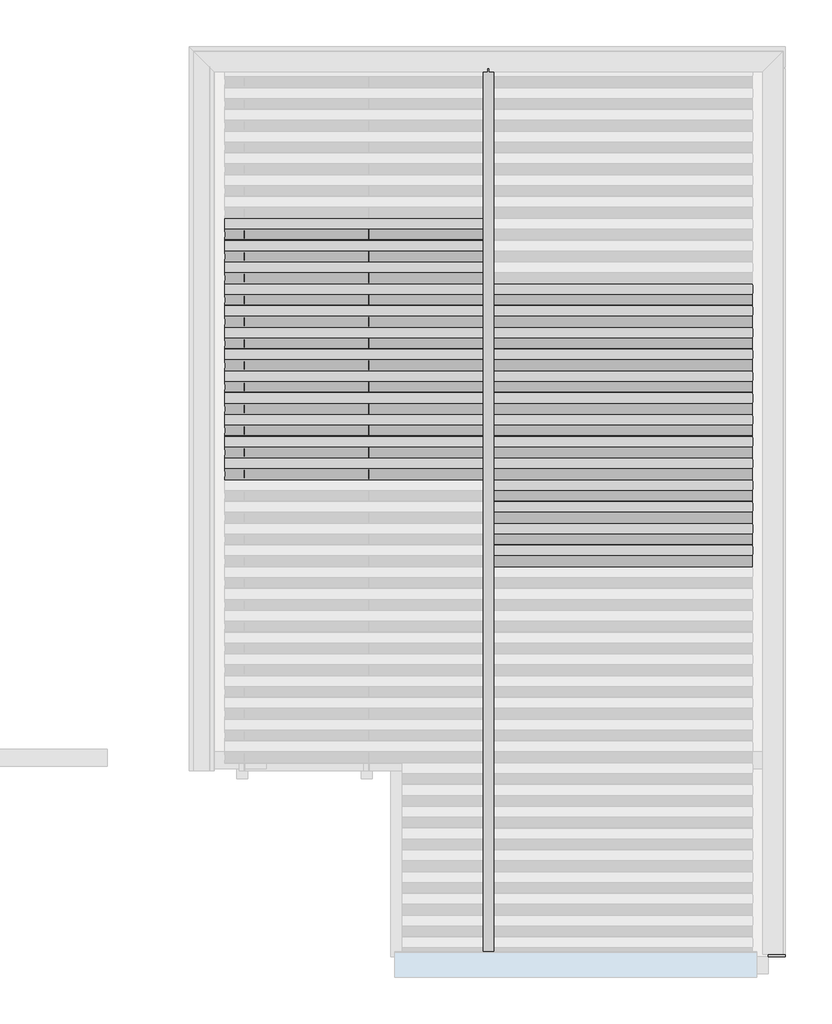
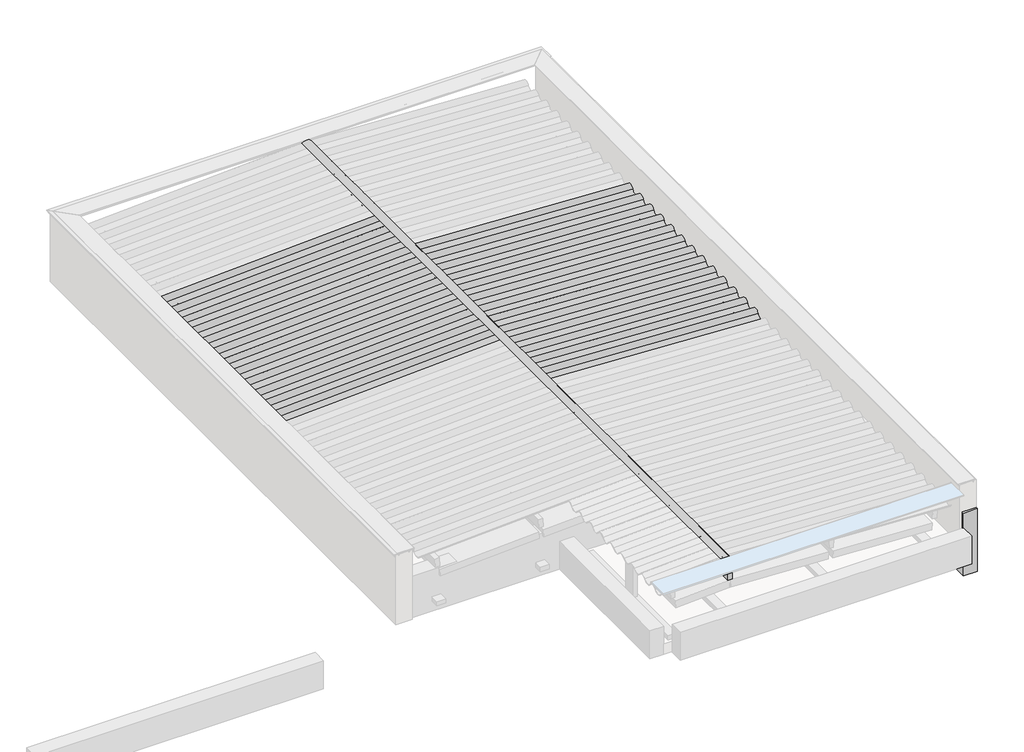
# One storey, part 3 of 4: 37 beams, 8 columns.
"""IFC4 building model written with IfcOpenShell, lengths in millimetres."""

import ifcopenshell
import ifcopenshell.guid

model = None  # the IFC model being written
_history = None  # IfcOwnerHistory: only IFC2X3 demands one
_inside = {}  # id of a spatial element -> (the spatial element, [elements in it])
_under = {}  # id of a project, library or spatial element -> (it, [spatial elements below it])
_declared = {}  # id of a project -> (the project, [libraries it declares])
_typed = {}  # id of a type object -> (the type object, [elements of that type])
_made_of = {}  # id of a material, layer set ... -> (it, [elements and type objects made of it])


def new_model(schema):
    """Start an empty IFC model of exactly this schema.

    Asked for "IFC4X3", IfcOpenShell would pick the latest addendum, in which some entities
    have other attributes; the version numbers below select the first issue.
    IFC2X3 requires an IfcOwnerHistory on every rooted entity: one is made here for all.
    """
    global model, _history
    if schema == "IFC4X3":
        model = ifcopenshell.file(schema_version=(4, 3, 0, 0))
    else:
        model = ifcopenshell.file(schema=schema)
    _inside.clear()
    _under.clear()
    _declared.clear()
    _typed.clear()
    _made_of.clear()
    _history = None
    if model.schema == "IFC2X3":
        org = make("IfcOrganization", Name="unknown")
        user = make(
            "IfcPersonAndOrganization",
            ThePerson=make("IfcPerson", FamilyName="unknown"),
            TheOrganization=org,
        )
        app = make(
            "IfcApplication",
            ApplicationDeveloper=org,
            Version="unknown",
            ApplicationFullName="unknown",
            ApplicationIdentifier="unknown",
        )
        _history = make(
            "IfcOwnerHistory",
            OwningUser=user,
            OwningApplication=app,
            ChangeAction="ADDED",
            CreationDate=0,
        )
    return model


def make(cls, **values):
    """One entity of the class cls with the attributes given. An attribute that is None is left unset."""
    return model.create_entity(
        cls, **{name: value for name, value in values.items() if value is not None}
    )


def rooted(cls, **values):
    """An entity with a GlobalId (a new one), such as an element, a storey or a relation."""
    return make(cls, GlobalId=ifcopenshell.guid.new(), OwnerHistory=_history, **values)


def si_unit(unit_type, name, prefix=None):
    """IfcSIUnit, for example si_unit("LENGTHUNIT", "METRE", prefix="MILLI")."""
    return make("IfcSIUnit", UnitType=unit_type, Prefix=prefix, Name=name)


def assignment(units):
    """IfcUnitAssignment: the units of a project."""
    return None if units is None else make("IfcUnitAssignment", Units=units)


def point(xyz):
    """IfcCartesianPoint."""
    return None if xyz is None else make("IfcCartesianPoint", Coordinates=xyz)


def direction(xyz):
    """IfcDirection."""
    return None if xyz is None else make("IfcDirection", DirectionRatios=xyz)


def frame(location, z_axis=None, x_axis=None):
    """IfcAxis2Placement3D, a coordinate frame: its origin and axes. An axis left out is left unset."""
    return make(
        "IfcAxis2Placement3D",
        Location=point(location),
        Axis=direction(z_axis),
        RefDirection=direction(x_axis),
    )


def frame_2d(location, x_axis=None):
    """IfcAxis2Placement2D, a coordinate frame in the plane: its origin and x axis."""
    return make(
        "IfcAxis2Placement2D", Location=point(location), RefDirection=direction(x_axis)
    )


def origin():
    """The frame at (0, 0, 0) with its axes left unset."""
    return frame((0.0, 0.0, 0.0))


def place(relative_to, where):
    """IfcLocalPlacement: puts the frame where relative to a parent placement (None: the world)."""
    return make(
        "IfcLocalPlacement", PlacementRelTo=relative_to, RelativePlacement=where
    )


def context(
    kind, dimensions, precision=None, world=None, true_north=None, identifier=None
):
    """IfcGeometricRepresentationContext, for example the 3D "Model" context."""
    return make(
        "IfcGeometricRepresentationContext",
        ContextIdentifier=identifier,
        ContextType=kind,
        CoordinateSpaceDimension=dimensions,
        Precision=precision,
        WorldCoordinateSystem=world,
        TrueNorth=true_north,
    )


def project(units=None, contexts=None):
    """IfcProject with its units and contexts."""
    return rooted(
        "IfcProject",
        Name="project",
        RepresentationContexts=contexts,
        UnitsInContext=assignment(units),
    )


def spatial(cls, under=None, at=None, **own):
    """A site, building, storey or space (cls), placed at a placement, below another one or the project."""
    s = rooted(cls, ObjectPlacement=at, **own)
    if under is not None:
        _under.setdefault(under.id(), (under, []))[1].append(s)
    return s


def polyline(points):
    """IfcPolyline through the points."""
    return make("IfcPolyline", Points=[point(p) for p in points])


def circle_curve(where, radius):
    """IfcCircle in the frame where."""
    return make("IfcCircle", Position=where, Radius=radius)


def trimmed(basis, trim1, trim2, sense, master):
    """IfcTrimmedCurve: the piece of a basis curve between two trims."""
    return make(
        "IfcTrimmedCurve",
        BasisCurve=basis,
        Trim1=trim1,
        Trim2=trim2,
        SenseAgreement=sense,
        MasterRepresentation=master,
    )


def segment(curve, same_sense, transition):
    """IfcCompositeCurveSegment."""
    return make(
        "IfcCompositeCurveSegment",
        Transition=transition,
        SameSense=same_sense,
        ParentCurve=curve,
    )


def composite_curve(segments, self_intersect=None):
    """IfcCompositeCurve: segments joined end to end."""
    return make("IfcCompositeCurve", Segments=segments, SelfIntersect=self_intersect)


def outline(outer, holes=None, kind="AREA"):
    """IfcArbitraryClosedProfileDef: a profile drawn as a closed curve; with holes, ...WithVoids."""
    if holes is None:
        return make("IfcArbitraryClosedProfileDef", ProfileType=kind, OuterCurve=outer)
    return make(
        "IfcArbitraryProfileDefWithVoids",
        ProfileType=kind,
        OuterCurve=outer,
        InnerCurves=holes,
    )


def extrude(swept, where, along, depth):
    """IfcExtrudedAreaSolid: the profile swept, set in the frame where, extruded along a direction by depth."""
    return make(
        "IfcExtrudedAreaSolid",
        SweptArea=swept,
        Position=where,
        ExtrudedDirection=direction(along),
        Depth=depth,
    )


def faces_of(points, faces, orient=None, outer=None):
    """IfcFace entities. A face is a list of loops; a loop is a list of indices into points, from 0.

    orient and outer hold one flag for each loop. By default every Orientation is true, the
    first loop of a face is its IfcFaceOuterBound and the others are IfcFaceBound.
    """
    made = []
    for i, loops in enumerate(faces):
        bounds = []
        for j, loop in enumerate(loops):
            is_outer = j == 0 if outer is None else outer[i][j]
            bounds.append(
                make(
                    "IfcFaceOuterBound" if is_outer else "IfcFaceBound",
                    Bound=make("IfcPolyLoop", Polygon=[points[k] for k in loop]),
                    Orientation=True if orient is None else orient[i][j],
                )
            )
        made.append(make("IfcFace", Bounds=bounds))
    return made


def faceted_brep(points, faces, orient=None, outer=None, voids=None):
    """IfcFacetedBrep: a solid bounded by flat faces; with voids (closed shells), ...WithVoids."""
    shared = [point(p) for p in points]
    hull = make("IfcClosedShell", CfsFaces=faces_of(shared, faces, orient, outer))
    if voids is None:
        return make("IfcFacetedBrep", Outer=hull)
    return make(
        "IfcFacetedBrepWithVoids",
        Outer=hull,
        Voids=[
            make(cls, CfsFaces=faces_of(shared, fs, o, b)) for cls, fs, o, b in voids
        ],
    )


def shape(context_of_items, identifier, shape_type, items):
    """IfcShapeRepresentation: the items that make up one representation, for example the "Body"."""
    return make(
        "IfcShapeRepresentation",
        ContextOfItems=context_of_items,
        RepresentationIdentifier=identifier,
        RepresentationType=shape_type,
        Items=items,
    )


def source(mapping_origin, context_of_items, identifier, shape_type, items):
    """IfcRepresentationMap: a shape defined once, which mapped items show again and again."""
    return make(
        "IfcRepresentationMap",
        MappingOrigin=mapping_origin,
        MappedRepresentation=shape(context_of_items, identifier, shape_type, items),
    )


def transform(
    local_origin,
    x_axis=None,
    y_axis=None,
    z_axis=None,
    scale=None,
    scale2=None,
    scale3=None,
    uniform=True,
):
    """IfcCartesianTransformationOperator3D, or its non-uniform kind. x_axis, y_axis, z_axis: its Axis1, 2, 3."""
    if uniform:
        return make(
            "IfcCartesianTransformationOperator3D",
            Axis1=direction(x_axis),
            Axis2=direction(y_axis),
            LocalOrigin=point(local_origin),
            Scale=scale,
            Axis3=direction(z_axis),
        )
    return make(
        "IfcCartesianTransformationOperator3DnonUniform",
        Axis1=direction(x_axis),
        Axis2=direction(y_axis),
        LocalOrigin=point(local_origin),
        Scale=scale,
        Axis3=direction(z_axis),
        Scale2=scale2,
        Scale3=scale3,
    )


def mapped(mapping_source, mapping_target):
    """IfcMappedItem: shows the shape of a source again, moved by a transform."""
    return make(
        "IfcMappedItem", MappingSource=mapping_source, MappingTarget=mapping_target
    )


def made_of(thing, what):
    """Note that an element or type object is made of a material, layer set ...; save() writes the relation."""
    if what is not None:
        _made_of.setdefault(what.id(), (what, []))[1].append(thing)
    return thing


def element(
    cls,
    number,
    at=None,
    inside=None,
    cuts=None,
    type_object=None,
    material=None,
    context=None,
    identifier="Body",
    shape_type=None,
    held_by="IfcProductDefinitionShape",
    body=None,
    shapes=None,
    **own,
):
    """One element of the class cls, such as IfcWall. Its Tag is "e" and its number.

    at: its placement. inside: the storey or other place that contains it. cuts: it is an
    opening in that element (IfcRelVoidsElement). A single representation is given by context,
    identifier, shape_type and body (its items); several are given by shapes. held_by: the class
    of the entity that holds the representations. save() writes the other relations.
    """
    e = rooted(cls, Tag="e%d" % number, ObjectPlacement=at, **own)
    if body is not None:
        shapes = [shape(context, identifier, shape_type, body)]
    if shapes is not None:
        e.Representation = make(held_by, Representations=shapes)
    if inside is not None:
        _inside.setdefault(inside.id(), (inside, []))[1].append(e)
    if cuts is not None:
        rooted(
            "IfcRelVoidsElement", RelatingBuildingElement=cuts, RelatedOpeningElement=e
        )
    if type_object is not None:
        _typed.setdefault(type_object.id(), (type_object, []))[1].append(e)
    return made_of(e, material)


def aggregate(whole, parts):
    """IfcRelAggregates: a whole, such as a stair, and the parts it consists of."""
    return rooted("IfcRelAggregates", RelatingObject=whole, RelatedObjects=parts)


def save(model, path):
    """Write the relations noted so far, then the file.

    IfcRelAggregates (storeys below a building ...), IfcRelContainedInSpatialStructure (elements
    in a storey), IfcRelDefinesByType, IfcRelAssociatesMaterial and IfcRelDeclares: one each for
    every whole, place, type object, material and project.
    """
    for whole, parts in _under.values():
        aggregate(whole, parts)
    for where, things in _inside.values():
        rooted(
            "IfcRelContainedInSpatialStructure",
            RelatedElements=things,
            RelatingStructure=where,
        )
    for kind, things in _typed.values():
        rooted("IfcRelDefinesByType", RelatedObjects=things, RelatingType=kind)
    for what, things in _made_of.values():
        rooted("IfcRelAssociatesMaterial", RelatedObjects=things, RelatingMaterial=what)
    for by, libraries in _declared.values():
        rooted("IfcRelDeclares", RelatingContext=by, RelatedDefinitions=libraries)
    model.write(path)


def cumeeira_telha_ondulada_fibrocimento_c9eafb3e(model_context):
    return source(origin(), model_context, "Body", "SweptSolid", [
        extrude(outline(composite_curve([segment(polyline([(58.3970135, 42.4437972), (53.9055884, 40.2467307)]), True, "CONTINUOUS"), segment(trimmed(circle_curve(frame_2d((-1.6029865, 13.0936483)), 61.7939461), [point((53.9055884, 40.2467307))], [point((-57.1115615, 40.2467307))], True, "CARTESIAN"), True, "CONTINUOUS"), segment(polyline([(-57.1115615, 40.2467307), (-61.6029865, 42.4437972)]), True, "CONTINUOUS"), segment(trimmed(circle_curve(frame_2d((-1.6029865, 13.0936483)), 66.7939461), [point((-61.6029865, 42.4437972))], [point((58.3970135, 42.4437972))], False, "CARTESIAN"), True, "CONTINUOUS")], self_intersect=False)), frame((-4969.5, 0.0, 0.0), z_axis=(1.0, 0.0, 0.0), x_axis=(0.0, 1.0, 0.0)), (0.0, 0.0, 1.0), 9939.0),
    ])


def viga_cumeeira_6x16cm_5eb8e513(model_context):
    return source(origin(), model_context, "Body", "SweptSolid", [
        extrude(outline(polyline([(4969.5, 30.0), (4969.5, -30.0), (-4969.5, -30.0), (-4969.5, 30.0), (4969.5, 30.0)])), frame((0.0, 0.0, -80.0), z_axis=(0.0, 0.0, 1.0), x_axis=(1.0, 0.0, 0.0)), (0.0, 0.0, 1.0), 160.0),
    ])


def column_f3930958(model_context):
    return source(origin(), model_context, "Body", "SweptSolid", [
        extrude(outline(polyline([(30.0, 80.0), (30.0, -80.0), (-30.0, -80.0), (-30.0, 80.0), (30.0, 80.0)])), frame((0.0, 0.0, 4460.0), z_axis=(0.0, 0.0, 1.0), x_axis=(1.0, 0.0, 0.0)), (0.0, 0.0, 1.0), 522.9),
    ])


def column_4d3918cc(model_context):
    return source(origin(), model_context, "Body", "SweptSolid", [
        extrude(outline(polyline([(30.0, 80.0), (30.0, -80.0), (-30.0, -80.0), (-30.0, 80.0), (30.0, 80.0)])), frame((0.0, 0.0, 4460.0), z_axis=(0.0, 0.0, 1.0), x_axis=(1.0, 0.0, 0.0)), (0.0, 0.0, 1.0), 426.9),
    ])


def column_924cc83b(model_context):
    return source(origin(), model_context, "Body", "SweptSolid", [
        extrude(outline(polyline([(30.0, 80.0), (30.0, -80.0), (-30.0, -80.0), (-30.0, 80.0), (30.0, 80.0)])), frame((0.0, 0.0, 4460.0), z_axis=(0.0, 0.0, 1.0), x_axis=(1.0, 0.0, 0.0)), (0.0, 0.0, 1.0), 497.0),
    ])


model = new_model("IFC4")

# Units and contexts
model_context = context("Model", 3, world=origin())
ifc_project = project(units=[si_unit("LENGTHUNIT", "METRE", prefix="MILLI")], contexts=[model_context])

# Site, building, storey
site = spatial("IfcSite", under=ifc_project)
building = spatial("IfcBuilding", under=site)
storey = spatial("IfcBuildingStorey", under=building, Name="COB. SALA ESTAR", Elevation=4400.0)

# Beams
placement = place(None, origin())
element("IfcBeam", 1, ObjectType="Madeira de lei : Berço 6x12cm", at=placement, inside=storey, context=model_context, shape_type="SweptSolid", body=[
    extrude(outline(polyline([(-3400.781307, 1623.9300153), (-3280.781307, 1623.9300153), (-3280.781307, -376.0699847), (-3400.781307, -376.0699847), (-3400.781307, 1623.9300153)])), frame((0.0, 0.0, 4400.0), z_axis=(0.0, 0.0, 1.0), x_axis=(1.0, 0.0, 0.0)), (0.0, 0.0, 1.0), 60.0),
])
element("IfcBeam", 2, ObjectType="Madeira de lei : Berço 6x12cm", at=placement, inside=storey, context=model_context, shape_type="SweptSolid", body=[
    extrude(outline(polyline([(-3400.781307, 3623.9300153), (-3280.781307, 3623.9300153), (-3280.781307, 1623.9300153), (-3400.781307, 1623.9300153), (-3400.781307, 3623.9300153)])), frame((0.0, 0.0, 4400.0), z_axis=(0.0, 0.0, 1.0), x_axis=(1.0, 0.0, 0.0)), (0.0, 0.0, 1.0), 60.0),
])
element("IfcBeam", 3, ObjectType="Madeira de lei : Berço 6x12cm", at=placement, inside=storey, context=model_context, shape_type="SweptSolid", body=[
    extrude(outline(polyline([(-2032.4438771, 1623.9300153), (-1912.4438771, 1623.9300153), (-1912.4438771, -376.0699847), (-2032.4438771, -376.0699847), (-2032.4438771, 1623.9300153)])), frame((0.0, 0.0, 4400.0), z_axis=(0.0, 0.0, 1.0), x_axis=(1.0, 0.0, 0.0)), (0.0, 0.0, 1.0), 60.0),
])
element("IfcBeam", 4, ObjectType="Madeira de lei : Berço 6x12cm", at=placement, inside=storey, context=model_context, shape_type="SweptSolid", body=[
    extrude(outline(polyline([(-2032.4438771, 3623.9300153), (-1912.4438771, 3623.9300153), (-1912.4438771, 1623.9300153), (-2032.4438771, 1623.9300153), (-2032.4438771, 3623.9300153)])), frame((0.0, 0.0, 4400.0), z_axis=(0.0, 0.0, 1.0), x_axis=(1.0, 0.0, 0.0)), (0.0, 0.0, 1.0), 60.0),
])
element("IfcBeam", 5, ObjectType="Madeira de lei : Berço 6x12cm", at=placement, inside=storey, context=model_context, shape_type="SweptSolid", body=[
    extrude(outline(polyline([(-634.1438771, 1623.9300153), (-514.1438771, 1623.9300153), (-514.1438771, -376.0699847), (-634.1438771, -376.0699847), (-634.1438771, 1623.9300153)])), frame((0.0, 0.0, 4400.0), z_axis=(0.0, 0.0, 1.0), x_axis=(1.0, 0.0, 0.0)), (0.0, 0.0, 1.0), 60.0),
])
element("IfcBeam", 6, ObjectType="Madeira de lei : Berço 6x12cm", at=placement, inside=storey, context=model_context, shape_type="SweptSolid", body=[
    extrude(outline(polyline([(-634.1438771, 3623.9300153), (-514.1438771, 3623.9300153), (-514.1438771, 1623.9300153), (-634.1438771, 1623.9300153), (-634.1438771, 3623.9300153)])), frame((0.0, 0.0, 4400.0), z_axis=(0.0, 0.0, 1.0), x_axis=(1.0, 0.0, 0.0)), (0.0, 0.0, 1.0), 60.0),
])
element("IfcBeam", 7, ObjectType="Madeira de lei : Berço 6x12cm", at=placement, inside=storey, context=model_context, shape_type="SweptSolid", body=[
    extrude(outline(polyline([(-4769.1187368, 1623.9300153), (-4649.1187368, 1623.9300153), (-4649.1187368, -376.0699847), (-4769.1187368, -376.0699847), (-4769.1187368, 1623.9300153)])), frame((0.0, 0.0, 4400.0), z_axis=(0.0, 0.0, 1.0), x_axis=(1.0, 0.0, 0.0)), (0.0, 0.0, 1.0), 60.0),
])
element("IfcBeam", 8, ObjectType="Madeira de lei : Berço 6x12cm", at=placement, inside=storey, context=model_context, shape_type="SweptSolid", body=[
    extrude(outline(polyline([(-4769.1187368, 3623.9300153), (-4649.1187368, 3623.9300153), (-4649.1187368, 1623.9300153), (-4769.1187368, 1623.9300153), (-4769.1187368, 3623.9300153)])), frame((0.0, 0.0, 4400.0), z_axis=(0.0, 0.0, 1.0), x_axis=(1.0, 0.0, 0.0)), (0.0, 0.0, 1.0), 60.0),
])
element("IfcBeam", 9, ObjectType="Madeira de lei : Berço 6x12cm", at=placement, inside=storey, context=model_context, shape_type="SweptSolid", body=[
    extrude(outline(polyline([(-6167.4187368, 3623.9300153), (-6047.4187368, 3623.9300153), (-6047.4187368, 1623.9300153), (-6167.4187368, 1623.9300153), (-6167.4187368, 3623.9300153)])), frame((0.0, 0.0, 4400.0), z_axis=(0.0, 0.0, 1.0), x_axis=(1.0, 0.0, 0.0)), (0.0, 0.0, 1.0), 60.0),
])
cumeeira_telha_ondulada_fibrocimento_shape = cumeeira_telha_ondulada_fibrocimento_c9eafb3e(model_context)
element("IfcBeam", 10, ObjectType="Cumeeira Telha Ondulada : Fibrocimento", at=placement, inside=storey, context=model_context, shape_type="MappedRepresentation", body=[
    mapped(cumeeira_telha_ondulada_fibrocimento_shape, transform((-3340.781307, 623.9300153, 5182.0251229), x_axis=(0.0, -1.0, 0.0), y_axis=(1.0, 0.0, 0.0), z_axis=(0.0, 0.0, 1.0))),
])
element("IfcBeam", 11, ObjectType="TQS - Viga retangular : 19.0 x 90.0", at=placement, inside=storey, context=model_context, shape_type="Brep", body=[
    faceted_brep([(-12.281307, 5584.4300153, 4850.0), (-202.2813068, 5584.4382679, 4850.0), (-202.6137562, -2069.5699847, 4850.0), (-202.6220088, -2259.5699847, 4850.0), (-202.7139163, -4375.561732, 4850.0), (-12.7139164, -4375.5699846, 4850.0), (-12.281307, 5584.4300153, 3950.0), (-12.7139164, -4375.5699846, 3950.0), (-202.2813068, 5584.4382679, 3950.0), (-202.7139163, -4375.561732, 3950.0)], [[[0, 1, 2, 3, 4, 5]], [[6, 0, 5, 7]], [[8, 6, 7, 9]], [[1, 8, 9, 4, 3, 2]], [[1, 0, 6, 8]], [[4, 9, 7, 5]]]),
])
element("IfcBeam", 12, ObjectType="Telha Ondulada : Fibrocimento", at=placement, inside=storey, context=model_context, shape_type="SweptSolid", body=[
    extrude(outline(composite_curve([segment(trimmed(circle_curve(frame_2d((-58.7002978, -53.2060538)), 66.7939461), [point((-29.3501488, 6.7939462))], [point((-29.3501488, -113.2060538))], False, "CARTESIAN"), True, "CONTINUOUS"), segment(polyline([(-29.3501488, -113.2060538), (-31.5472154, -108.7146288)]), True, "CONTINUOUS"), segment(trimmed(circle_curve(frame_2d((-58.7002978, -53.2060538)), 61.7939461), [point((-31.5472154, -108.7146288))], [point((-31.5472154, 2.3025211))], True, "CARTESIAN"), True, "CONTINUOUS"), segment(trimmed(circle_curve(frame_2d((0.0, 66.7939462)), 71.7939461), [point((-31.5472154, 2.3025211))], [point((-31.5472154, 131.2853712))], False, "CARTESIAN"), True, "CONTINUOUS"), segment(polyline([(-31.5472154, 131.2853712), (-29.3501488, 126.7939462)]), True, "CONTINUOUS"), segment(trimmed(circle_curve(frame_2d((0.0, 66.7939462)), 66.7939461), [point((-29.3501488, 126.7939462))], [point((-29.3501488, 6.7939462))], True, "CARTESIAN"), True, "CONTINUOUS")], self_intersect=False)), frame((-6303.6781287, 1111.326948, 5068.1236978), z_axis=(0.9987523388778448, 0.0, 0.04993761694389136), x_axis=(-0.04993761694389136, 0.0, 0.9987523388778448)), (0.0, 0.0, 1.0), 2962.0084336),
])
element("IfcBeam", 13, ObjectType="Telha Ondulada : Fibrocimento", at=placement, inside=storey, context=model_context, shape_type="SweptSolid", body=[
    extrude(outline(composite_curve([segment(trimmed(circle_curve(frame_2d((-58.7002978, -53.2060538)), 66.7939461), [point((-29.3501488, 6.7939462))], [point((-29.3501488, -113.2060538))], False, "CARTESIAN"), True, "CONTINUOUS"), segment(polyline([(-29.3501488, -113.2060538), (-31.5472154, -108.7146288)]), True, "CONTINUOUS"), segment(trimmed(circle_curve(frame_2d((-58.7002978, -53.2060538)), 61.7939461), [point((-31.5472154, -108.7146288))], [point((-31.5472154, 2.3025211))], True, "CARTESIAN"), True, "CONTINUOUS"), segment(trimmed(circle_curve(frame_2d((0.0, 66.7939462)), 71.7939461), [point((-31.5472154, 2.3025211))], [point((-31.5472154, 131.2853712))], False, "CARTESIAN"), True, "CONTINUOUS"), segment(polyline([(-31.5472154, 131.2853712), (-29.3501488, 126.7939462)]), True, "CONTINUOUS"), segment(trimmed(circle_curve(frame_2d((0.0, 66.7939462)), 66.7939461), [point((-29.3501488, 126.7939462))], [point((-29.3501488, 6.7939462))], True, "CARTESIAN"), True, "CONTINUOUS")], self_intersect=False)), frame((-6303.6781287, 1355.826948, 5068.1236978), z_axis=(0.9987523388778448, 0.0, 0.04993761694389134), x_axis=(-0.04993761694389134, 0.0, 0.9987523388778448)), (0.0, 0.0, 1.0), 2962.0084336),
])
element("IfcBeam", 14, ObjectType="Telha Ondulada : Fibrocimento", at=placement, inside=storey, context=model_context, shape_type="SweptSolid", body=[
    extrude(outline(composite_curve([segment(trimmed(circle_curve(frame_2d((-58.7002978, -53.2060538)), 66.7939461), [point((-29.3501488, 6.7939462))], [point((-29.3501488, -113.2060538))], False, "CARTESIAN"), True, "CONTINUOUS"), segment(polyline([(-29.3501488, -113.2060538), (-31.5472154, -108.7146288)]), True, "CONTINUOUS"), segment(trimmed(circle_curve(frame_2d((-58.7002978, -53.2060538)), 61.7939461), [point((-31.5472154, -108.7146288))], [point((-31.5472154, 2.3025211))], True, "CARTESIAN"), True, "CONTINUOUS"), segment(trimmed(circle_curve(frame_2d((0.0, 66.7939462)), 71.7939461), [point((-31.5472154, 2.3025211))], [point((-31.5472154, 131.2853712))], False, "CARTESIAN"), True, "CONTINUOUS"), segment(polyline([(-31.5472154, 131.2853712), (-29.3501488, 126.7939462)]), True, "CONTINUOUS"), segment(trimmed(circle_curve(frame_2d((0.0, 66.7939462)), 66.7939461), [point((-29.3501488, 126.7939462))], [point((-29.3501488, 6.7939462))], True, "CARTESIAN"), True, "CONTINUOUS")], self_intersect=False)), frame((-6303.6781287, 1600.326948, 5068.1236978), z_axis=(0.9987523388778448, 0.0, 0.04993761694389136), x_axis=(-0.04993761694389136, 0.0, 0.9987523388778448)), (0.0, 0.0, 1.0), 2962.0084336),
])
element("IfcBeam", 15, ObjectType="Telha Ondulada : Fibrocimento", at=placement, inside=storey, context=model_context, shape_type="SweptSolid", body=[
    extrude(outline(composite_curve([segment(trimmed(circle_curve(frame_2d((-58.7002978, -53.2060538)), 66.7939461), [point((-29.3501488, 6.7939462))], [point((-29.3501488, -113.2060538))], False, "CARTESIAN"), True, "CONTINUOUS"), segment(polyline([(-29.3501488, -113.2060538), (-31.5472154, -108.7146288)]), True, "CONTINUOUS"), segment(trimmed(circle_curve(frame_2d((-58.7002978, -53.2060538)), 61.7939461), [point((-31.5472154, -108.7146288))], [point((-31.5472154, 2.3025211))], True, "CARTESIAN"), True, "CONTINUOUS"), segment(trimmed(circle_curve(frame_2d((0.0, 66.7939462)), 71.7939461), [point((-31.5472154, 2.3025211))], [point((-31.5472154, 131.2853712))], False, "CARTESIAN"), True, "CONTINUOUS"), segment(polyline([(-31.5472154, 131.2853712), (-29.3501488, 126.7939462)]), True, "CONTINUOUS"), segment(trimmed(circle_curve(frame_2d((0.0, 66.7939462)), 66.7939461), [point((-29.3501488, 126.7939462))], [point((-29.3501488, 6.7939462))], True, "CARTESIAN"), True, "CONTINUOUS")], self_intersect=False)), frame((-6303.6781287, 1844.826948, 5068.1236978), z_axis=(0.9987523388778448, 0.0, 0.049937616943891344), x_axis=(-0.049937616943891344, 0.0, 0.9987523388778448)), (0.0, 0.0, 1.0), 2962.0084336),
])
element("IfcBeam", 16, ObjectType="Telha Ondulada : Fibrocimento", at=placement, inside=storey, context=model_context, shape_type="SweptSolid", body=[
    extrude(outline(composite_curve([segment(trimmed(circle_curve(frame_2d((-58.7002978, -53.2060538)), 66.7939461), [point((-29.3501488, 6.7939462))], [point((-29.3501488, -113.2060538))], False, "CARTESIAN"), True, "CONTINUOUS"), segment(polyline([(-29.3501488, -113.2060538), (-31.5472154, -108.7146288)]), True, "CONTINUOUS"), segment(trimmed(circle_curve(frame_2d((-58.7002978, -53.2060538)), 61.7939461), [point((-31.5472154, -108.7146288))], [point((-31.5472154, 2.3025211))], True, "CARTESIAN"), True, "CONTINUOUS"), segment(trimmed(circle_curve(frame_2d((0.0, 66.7939462)), 71.7939461), [point((-31.5472154, 2.3025211))], [point((-31.5472154, 131.2853712))], False, "CARTESIAN"), True, "CONTINUOUS"), segment(polyline([(-31.5472154, 131.2853712), (-29.3501488, 126.7939462)]), True, "CONTINUOUS"), segment(trimmed(circle_curve(frame_2d((0.0, 66.7939462)), 66.7939461), [point((-29.3501488, 126.7939462))], [point((-29.3501488, 6.7939462))], True, "CARTESIAN"), True, "CONTINUOUS")], self_intersect=False)), frame((-6303.6781287, 2089.326948, 5068.1236978), z_axis=(0.9987523388778448, 0.0, 0.04993761694389134), x_axis=(-0.04993761694389134, 0.0, 0.9987523388778448)), (0.0, 0.0, 1.0), 2962.0084336),
])
element("IfcBeam", 17, ObjectType="Telha Ondulada : Fibrocimento", at=placement, inside=storey, context=model_context, shape_type="SweptSolid", body=[
    extrude(outline(composite_curve([segment(trimmed(circle_curve(frame_2d((-58.7002978, -53.2060538)), 66.7939461), [point((-29.3501488, 6.7939462))], [point((-29.3501488, -113.2060538))], False, "CARTESIAN"), True, "CONTINUOUS"), segment(polyline([(-29.3501488, -113.2060538), (-31.5472154, -108.7146288)]), True, "CONTINUOUS"), segment(trimmed(circle_curve(frame_2d((-58.7002978, -53.2060538)), 61.7939461), [point((-31.5472154, -108.7146288))], [point((-31.5472154, 2.3025211))], True, "CARTESIAN"), True, "CONTINUOUS"), segment(trimmed(circle_curve(frame_2d((0.0, 66.7939462)), 71.7939461), [point((-31.5472154, 2.3025211))], [point((-31.5472154, 131.2853712))], False, "CARTESIAN"), True, "CONTINUOUS"), segment(polyline([(-31.5472154, 131.2853712), (-29.3501488, 126.7939462)]), True, "CONTINUOUS"), segment(trimmed(circle_curve(frame_2d((0.0, 66.7939462)), 66.7939461), [point((-29.3501488, 126.7939462))], [point((-29.3501488, 6.7939462))], True, "CARTESIAN"), True, "CONTINUOUS")], self_intersect=False)), frame((-6303.6781287, 2333.826948, 5068.1236978), z_axis=(0.9987523388778448, 0.0, 0.04993761694389136), x_axis=(-0.04993761694389136, 0.0, 0.9987523388778448)), (0.0, 0.0, 1.0), 2962.0084336),
])
element("IfcBeam", 18, ObjectType="Telha Ondulada : Fibrocimento", at=placement, inside=storey, context=model_context, shape_type="SweptSolid", body=[
    extrude(outline(composite_curve([segment(trimmed(circle_curve(frame_2d((-58.7002978, -53.2060538)), 66.7939461), [point((-29.3501488, 6.7939462))], [point((-29.3501488, -113.2060538))], False, "CARTESIAN"), True, "CONTINUOUS"), segment(polyline([(-29.3501488, -113.2060538), (-31.5472154, -108.7146288)]), True, "CONTINUOUS"), segment(trimmed(circle_curve(frame_2d((-58.7002978, -53.2060538)), 61.7939461), [point((-31.5472154, -108.7146288))], [point((-31.5472154, 2.3025211))], True, "CARTESIAN"), True, "CONTINUOUS"), segment(trimmed(circle_curve(frame_2d((0.0, 66.7939462)), 71.7939461), [point((-31.5472154, 2.3025211))], [point((-31.5472154, 131.2853712))], False, "CARTESIAN"), True, "CONTINUOUS"), segment(polyline([(-31.5472154, 131.2853712), (-29.3501488, 126.7939462)]), True, "CONTINUOUS"), segment(trimmed(circle_curve(frame_2d((0.0, 66.7939462)), 66.7939461), [point((-29.3501488, 126.7939462))], [point((-29.3501488, 6.7939462))], True, "CARTESIAN"), True, "CONTINUOUS")], self_intersect=False)), frame((-6303.6781287, 2578.326948, 5068.1236978), z_axis=(0.9987523388778448, 0.0, 0.04993761694389134), x_axis=(-0.04993761694389134, 0.0, 0.9987523388778448)), (0.0, 0.0, 1.0), 2962.0084336),
])
element("IfcBeam", 19, ObjectType="Telha Ondulada : Fibrocimento", at=placement, inside=storey, context=model_context, shape_type="SweptSolid", body=[
    extrude(outline(composite_curve([segment(trimmed(circle_curve(frame_2d((-58.7002978, -53.2060538)), 66.7939461), [point((-29.3501488, 6.7939462))], [point((-29.3501488, -113.2060538))], False, "CARTESIAN"), True, "CONTINUOUS"), segment(polyline([(-29.3501488, -113.2060538), (-31.5472154, -108.7146288)]), True, "CONTINUOUS"), segment(trimmed(circle_curve(frame_2d((-58.7002978, -53.2060538)), 61.7939461), [point((-31.5472154, -108.7146288))], [point((-31.5472154, 2.3025211))], True, "CARTESIAN"), True, "CONTINUOUS"), segment(trimmed(circle_curve(frame_2d((0.0, 66.7939462)), 71.7939461), [point((-31.5472154, 2.3025211))], [point((-31.5472154, 131.2853712))], False, "CARTESIAN"), True, "CONTINUOUS"), segment(polyline([(-31.5472154, 131.2853712), (-29.3501488, 126.7939462)]), True, "CONTINUOUS"), segment(trimmed(circle_curve(frame_2d((0.0, 66.7939462)), 66.7939461), [point((-29.3501488, 126.7939462))], [point((-29.3501488, 6.7939462))], True, "CARTESIAN"), True, "CONTINUOUS")], self_intersect=False)), frame((-6303.6781287, 2822.826948, 5068.1236978), z_axis=(0.9987523388778448, 0.0, 0.04993761694389136), x_axis=(-0.04993761694389136, 0.0, 0.9987523388778448)), (0.0, 0.0, 1.0), 2962.0084336),
])
element("IfcBeam", 20, ObjectType="Telha Ondulada : Fibrocimento", at=placement, inside=storey, context=model_context, shape_type="SweptSolid", body=[
    extrude(outline(composite_curve([segment(trimmed(circle_curve(frame_2d((-58.7002978, -53.2060538)), 66.7939461), [point((-29.3501488, 6.7939462))], [point((-29.3501488, -113.2060538))], False, "CARTESIAN"), True, "CONTINUOUS"), segment(polyline([(-29.3501488, -113.2060538), (-31.5472154, -108.7146288)]), True, "CONTINUOUS"), segment(trimmed(circle_curve(frame_2d((-58.7002978, -53.2060538)), 61.7939461), [point((-31.5472154, -108.7146288))], [point((-31.5472154, 2.3025211))], True, "CARTESIAN"), True, "CONTINUOUS"), segment(trimmed(circle_curve(frame_2d((0.0, 66.7939462)), 71.7939461), [point((-31.5472154, 2.3025211))], [point((-31.5472154, 131.2853712))], False, "CARTESIAN"), True, "CONTINUOUS"), segment(polyline([(-31.5472154, 131.2853712), (-29.3501488, 126.7939462)]), True, "CONTINUOUS"), segment(trimmed(circle_curve(frame_2d((0.0, 66.7939462)), 66.7939461), [point((-29.3501488, 126.7939462))], [point((-29.3501488, 6.7939462))], True, "CARTESIAN"), True, "CONTINUOUS")], self_intersect=False)), frame((-6303.6781287, 3067.326948, 5068.1236978), z_axis=(0.9987523388778448, 0.0, 0.04993761694389134), x_axis=(-0.04993761694389134, 0.0, 0.9987523388778448)), (0.0, 0.0, 1.0), 2962.0084336),
])
element("IfcBeam", 21, ObjectType="Telha Ondulada : Fibrocimento", at=placement, inside=storey, context=model_context, shape_type="SweptSolid", body=[
    extrude(outline(composite_curve([segment(trimmed(circle_curve(frame_2d((-58.7002978, -53.2060538)), 66.7939461), [point((-29.3501488, 6.7939462))], [point((-29.3501488, -113.2060538))], False, "CARTESIAN"), True, "CONTINUOUS"), segment(polyline([(-29.3501488, -113.2060538), (-31.5472154, -108.7146288)]), True, "CONTINUOUS"), segment(trimmed(circle_curve(frame_2d((-58.7002978, -53.2060538)), 61.7939461), [point((-31.5472154, -108.7146288))], [point((-31.5472154, 2.3025211))], True, "CARTESIAN"), True, "CONTINUOUS"), segment(trimmed(circle_curve(frame_2d((0.0, 66.7939462)), 71.7939461), [point((-31.5472154, 2.3025211))], [point((-31.5472154, 131.2853712))], False, "CARTESIAN"), True, "CONTINUOUS"), segment(polyline([(-31.5472154, 131.2853712), (-29.3501488, 126.7939462)]), True, "CONTINUOUS"), segment(trimmed(circle_curve(frame_2d((0.0, 66.7939462)), 66.7939461), [point((-29.3501488, 126.7939462))], [point((-29.3501488, 6.7939462))], True, "CARTESIAN"), True, "CONTINUOUS")], self_intersect=False)), frame((-6303.6781287, 3311.826948, 5068.1236978), z_axis=(0.9987523388778448, 0.0, 0.04993761694389133), x_axis=(-0.04993761694389133, 0.0, 0.9987523388778448)), (0.0, 0.0, 1.0), 2962.0084336),
])
element("IfcBeam", 22, ObjectType="Telha Ondulada : Fibrocimento", at=placement, inside=storey, context=model_context, shape_type="SweptSolid", body=[
    extrude(outline(composite_curve([segment(trimmed(circle_curve(frame_2d((-58.7002978, -53.2060538)), 66.7939461), [point((-29.3501488, 6.7939462))], [point((-29.3501488, -113.2060538))], False, "CARTESIAN"), True, "CONTINUOUS"), segment(polyline([(-29.3501488, -113.2060538), (-31.5472154, -108.7146288)]), True, "CONTINUOUS"), segment(trimmed(circle_curve(frame_2d((-58.7002978, -53.2060538)), 61.7939461), [point((-31.5472154, -108.7146288))], [point((-31.5472154, 2.3025211))], True, "CARTESIAN"), True, "CONTINUOUS"), segment(trimmed(circle_curve(frame_2d((0.0, 66.7939462)), 71.7939461), [point((-31.5472154, 2.3025211))], [point((-31.5472154, 131.2853712))], False, "CARTESIAN"), True, "CONTINUOUS"), segment(polyline([(-31.5472154, 131.2853712), (-29.3501488, 126.7939462)]), True, "CONTINUOUS"), segment(trimmed(circle_curve(frame_2d((0.0, 66.7939462)), 66.7939461), [point((-29.3501488, 126.7939462))], [point((-29.3501488, 6.7939462))], True, "CARTESIAN"), True, "CONTINUOUS")], self_intersect=False)), frame((-6303.6781287, 3556.326948, 5068.1236978), z_axis=(0.9987523388778448, 0.0, 0.049937616943891344), x_axis=(-0.049937616943891344, 0.0, 0.9987523388778448)), (0.0, 0.0, 1.0), 2962.0084336),
])
element("IfcBeam", 23, ObjectType="Telha Ondulada : Fibrocimento", at=placement, inside=storey, context=model_context, shape_type="SweptSolid", body=[
    extrude(outline(composite_curve([segment(trimmed(circle_curve(frame_2d((-58.7002978, -53.2060538)), 66.7939461), [point((-29.3501488, 6.7939462))], [point((-29.3501488, -113.2060538))], False, "CARTESIAN"), True, "CONTINUOUS"), segment(polyline([(-29.3501488, -113.2060538), (-31.5472154, -108.7146288)]), True, "CONTINUOUS"), segment(trimmed(circle_curve(frame_2d((-58.7002978, -53.2060538)), 61.7939461), [point((-31.5472154, -108.7146288))], [point((-31.5472154, 2.3025211))], True, "CARTESIAN"), True, "CONTINUOUS"), segment(trimmed(circle_curve(frame_2d((0.0, 66.7939462)), 71.7939461), [point((-31.5472154, 2.3025211))], [point((-31.5472154, 131.2853712))], False, "CARTESIAN"), True, "CONTINUOUS"), segment(polyline([(-31.5472154, 131.2853712), (-29.3501488, 126.7939462)]), True, "CONTINUOUS"), segment(trimmed(circle_curve(frame_2d((0.0, 66.7939462)), 66.7939461), [point((-29.3501488, 126.7939462))], [point((-29.3501488, 6.7939462))], True, "CARTESIAN"), True, "CONTINUOUS")], self_intersect=False)), frame((-6303.6781287, 3800.826948, 5068.1236978), z_axis=(0.9987523388778448, 0.0, 0.04993761694389134), x_axis=(-0.04993761694389134, 0.0, 0.9987523388778448)), (0.0, 0.0, 1.0), 2962.0084336),
])
element("IfcBeam", 24, ObjectType="Telha Ondulada : Fibrocimento", at=placement, inside=storey, context=model_context, shape_type="SweptSolid", body=[
    extrude(outline(composite_curve([segment(trimmed(circle_curve(frame_2d((0.0, 66.7939462)), 66.7939461), [point((29.3501488, 6.7939462))], [point((29.3501488, 126.7939462))], True, "CARTESIAN"), True, "CONTINUOUS"), segment(polyline([(29.3501488, 126.7939462), (31.5472154, 131.2853712)]), True, "CONTINUOUS"), segment(trimmed(circle_curve(frame_2d((0.0, 66.7939462)), 71.7939461), [point((31.5472154, 131.2853712))], [point((31.5472154, 2.3025211))], False, "CARTESIAN"), True, "CONTINUOUS"), segment(trimmed(circle_curve(frame_2d((58.7002978, -53.2060538)), 61.7939461), [point((31.5472154, 2.3025211))], [point((31.5472154, -108.7146288))], True, "CARTESIAN"), True, "CONTINUOUS"), segment(polyline([(31.5472154, -108.7146288), (29.3501488, -113.2060538)]), True, "CONTINUOUS"), segment(trimmed(circle_curve(frame_2d((58.7002978, -53.2060538)), 66.7939461), [point((29.3501488, -113.2060538))], [point((29.3501488, 6.7939462))], False, "CARTESIAN"), True, "CONTINUOUS")], self_intersect=False)), frame((-377.8844852, 133.326948, 5068.1236978), z_axis=(-0.9987523388778448, 0.0, 0.04993761694389145), x_axis=(-0.04993761694389145, 0.0, -0.9987523388778448)), (0.0, 0.0, 1.0), 2962.0084336),
])
element("IfcBeam", 25, ObjectType="Telha Ondulada : Fibrocimento", at=placement, inside=storey, context=model_context, shape_type="SweptSolid", body=[
    extrude(outline(composite_curve([segment(trimmed(circle_curve(frame_2d((0.0, 66.7939462)), 66.7939461), [point((29.3501488, 6.7939462))], [point((29.3501488, 126.7939462))], True, "CARTESIAN"), True, "CONTINUOUS"), segment(polyline([(29.3501488, 126.7939462), (31.5472154, 131.2853712)]), True, "CONTINUOUS"), segment(trimmed(circle_curve(frame_2d((0.0, 66.7939462)), 71.7939461), [point((31.5472154, 131.2853712))], [point((31.5472154, 2.3025211))], False, "CARTESIAN"), True, "CONTINUOUS"), segment(trimmed(circle_curve(frame_2d((58.7002978, -53.2060538)), 61.7939461), [point((31.5472154, 2.3025211))], [point((31.5472154, -108.7146288))], True, "CARTESIAN"), True, "CONTINUOUS"), segment(polyline([(31.5472154, -108.7146288), (29.3501488, -113.2060538)]), True, "CONTINUOUS"), segment(trimmed(circle_curve(frame_2d((58.7002978, -53.2060538)), 66.7939461), [point((29.3501488, -113.2060538))], [point((29.3501488, 6.7939462))], False, "CARTESIAN"), True, "CONTINUOUS")], self_intersect=False)), frame((-377.8844852, 377.826948, 5068.1236978), z_axis=(-0.9987523388778448, 0.0, 0.04993761694389145), x_axis=(-0.04993761694389145, 0.0, -0.9987523388778448)), (0.0, 0.0, 1.0), 2962.0084336),
])
element("IfcBeam", 26, ObjectType="Telha Ondulada : Fibrocimento", at=placement, inside=storey, context=model_context, shape_type="SweptSolid", body=[
    extrude(outline(composite_curve([segment(trimmed(circle_curve(frame_2d((0.0, 66.7939462)), 66.7939461), [point((29.3501488, 6.7939462))], [point((29.3501488, 126.7939462))], True, "CARTESIAN"), True, "CONTINUOUS"), segment(polyline([(29.3501488, 126.7939462), (31.5472154, 131.2853712)]), True, "CONTINUOUS"), segment(trimmed(circle_curve(frame_2d((0.0, 66.7939462)), 71.7939461), [point((31.5472154, 131.2853712))], [point((31.5472154, 2.3025211))], False, "CARTESIAN"), True, "CONTINUOUS"), segment(trimmed(circle_curve(frame_2d((58.7002978, -53.2060538)), 61.7939461), [point((31.5472154, 2.3025211))], [point((31.5472154, -108.7146288))], True, "CARTESIAN"), True, "CONTINUOUS"), segment(polyline([(31.5472154, -108.7146288), (29.3501488, -113.2060538)]), True, "CONTINUOUS"), segment(trimmed(circle_curve(frame_2d((58.7002978, -53.2060538)), 66.7939461), [point((29.3501488, -113.2060538))], [point((29.3501488, 6.7939462))], False, "CARTESIAN"), True, "CONTINUOUS")], self_intersect=False)), frame((-377.8844852, 622.326948, 5068.1236978), z_axis=(-0.9987523388778448, 0.0, 0.049937616943891455), x_axis=(-0.049937616943891455, 0.0, -0.9987523388778448)), (0.0, 0.0, 1.0), 2962.0084336),
])
element("IfcBeam", 27, ObjectType="Telha Ondulada : Fibrocimento", at=placement, inside=storey, context=model_context, shape_type="SweptSolid", body=[
    extrude(outline(composite_curve([segment(trimmed(circle_curve(frame_2d((0.0, 66.7939462)), 66.7939461), [point((29.3501488, 6.7939462))], [point((29.3501488, 126.7939462))], True, "CARTESIAN"), True, "CONTINUOUS"), segment(polyline([(29.3501488, 126.7939462), (31.5472154, 131.2853712)]), True, "CONTINUOUS"), segment(trimmed(circle_curve(frame_2d((0.0, 66.7939462)), 71.7939461), [point((31.5472154, 131.2853712))], [point((31.5472154, 2.3025211))], False, "CARTESIAN"), True, "CONTINUOUS"), segment(trimmed(circle_curve(frame_2d((58.7002978, -53.2060538)), 61.7939461), [point((31.5472154, 2.3025211))], [point((31.5472154, -108.7146288))], True, "CARTESIAN"), True, "CONTINUOUS"), segment(polyline([(31.5472154, -108.7146288), (29.3501488, -113.2060538)]), True, "CONTINUOUS"), segment(trimmed(circle_curve(frame_2d((58.7002978, -53.2060538)), 66.7939461), [point((29.3501488, -113.2060538))], [point((29.3501488, 6.7939462))], False, "CARTESIAN"), True, "CONTINUOUS")], self_intersect=False)), frame((-377.8844852, 866.826948, 5068.1236978), z_axis=(-0.9987523388778448, 0.0, 0.049937616943891455), x_axis=(-0.049937616943891455, 0.0, -0.9987523388778448)), (0.0, 0.0, 1.0), 2962.0084336),
])
element("IfcBeam", 28, ObjectType="Telha Ondulada : Fibrocimento", at=placement, inside=storey, context=model_context, shape_type="SweptSolid", body=[
    extrude(outline(composite_curve([segment(trimmed(circle_curve(frame_2d((0.0, 66.7939462)), 66.7939461), [point((29.3501488, 6.7939462))], [point((29.3501488, 126.7939462))], True, "CARTESIAN"), True, "CONTINUOUS"), segment(polyline([(29.3501488, 126.7939462), (31.5472154, 131.2853712)]), True, "CONTINUOUS"), segment(trimmed(circle_curve(frame_2d((0.0, 66.7939462)), 71.7939461), [point((31.5472154, 131.2853712))], [point((31.5472154, 2.3025211))], False, "CARTESIAN"), True, "CONTINUOUS"), segment(trimmed(circle_curve(frame_2d((58.7002978, -53.2060538)), 61.7939461), [point((31.5472154, 2.3025211))], [point((31.5472154, -108.7146288))], True, "CARTESIAN"), True, "CONTINUOUS"), segment(polyline([(31.5472154, -108.7146288), (29.3501488, -113.2060538)]), True, "CONTINUOUS"), segment(trimmed(circle_curve(frame_2d((58.7002978, -53.2060538)), 66.7939461), [point((29.3501488, -113.2060538))], [point((29.3501488, 6.7939462))], False, "CARTESIAN"), True, "CONTINUOUS")], self_intersect=False)), frame((-377.8844852, 1111.326948, 5068.1236978), z_axis=(-0.9987523388778448, 0.0, 0.049937616943891455), x_axis=(-0.049937616943891455, 0.0, -0.9987523388778448)), (0.0, 0.0, 1.0), 2962.0084336),
])
element("IfcBeam", 29, ObjectType="Telha Ondulada : Fibrocimento", at=placement, inside=storey, context=model_context, shape_type="SweptSolid", body=[
    extrude(outline(composite_curve([segment(trimmed(circle_curve(frame_2d((0.0, 66.7939462)), 66.7939461), [point((29.3501488, 6.7939462))], [point((29.3501488, 126.7939462))], True, "CARTESIAN"), True, "CONTINUOUS"), segment(polyline([(29.3501488, 126.7939462), (31.5472154, 131.2853712)]), True, "CONTINUOUS"), segment(trimmed(circle_curve(frame_2d((0.0, 66.7939462)), 71.7939461), [point((31.5472154, 131.2853712))], [point((31.5472154, 2.3025211))], False, "CARTESIAN"), True, "CONTINUOUS"), segment(trimmed(circle_curve(frame_2d((58.7002978, -53.2060538)), 61.7939461), [point((31.5472154, 2.3025211))], [point((31.5472154, -108.7146288))], True, "CARTESIAN"), True, "CONTINUOUS"), segment(polyline([(31.5472154, -108.7146288), (29.3501488, -113.2060538)]), True, "CONTINUOUS"), segment(trimmed(circle_curve(frame_2d((58.7002978, -53.2060538)), 66.7939461), [point((29.3501488, -113.2060538))], [point((29.3501488, 6.7939462))], False, "CARTESIAN"), True, "CONTINUOUS")], self_intersect=False)), frame((-377.8844852, 1355.826948, 5068.1236978), z_axis=(-0.9987523388778448, 0.0, 0.049937616943891455), x_axis=(-0.049937616943891455, 0.0, -0.9987523388778448)), (0.0, 0.0, 1.0), 2962.0084336),
])
element("IfcBeam", 30, ObjectType="Telha Ondulada : Fibrocimento", at=placement, inside=storey, context=model_context, shape_type="SweptSolid", body=[
    extrude(outline(composite_curve([segment(trimmed(circle_curve(frame_2d((0.0, 66.7939462)), 66.7939461), [point((29.3501488, 6.7939462))], [point((29.3501488, 126.7939462))], True, "CARTESIAN"), True, "CONTINUOUS"), segment(polyline([(29.3501488, 126.7939462), (31.5472154, 131.2853712)]), True, "CONTINUOUS"), segment(trimmed(circle_curve(frame_2d((0.0, 66.7939462)), 71.7939461), [point((31.5472154, 131.2853712))], [point((31.5472154, 2.3025211))], False, "CARTESIAN"), True, "CONTINUOUS"), segment(trimmed(circle_curve(frame_2d((58.7002978, -53.2060538)), 61.7939461), [point((31.5472154, 2.3025211))], [point((31.5472154, -108.7146288))], True, "CARTESIAN"), True, "CONTINUOUS"), segment(polyline([(31.5472154, -108.7146288), (29.3501488, -113.2060538)]), True, "CONTINUOUS"), segment(trimmed(circle_curve(frame_2d((58.7002978, -53.2060538)), 66.7939461), [point((29.3501488, -113.2060538))], [point((29.3501488, 6.7939462))], False, "CARTESIAN"), True, "CONTINUOUS")], self_intersect=False)), frame((-377.8844852, 1600.326948, 5068.1236978), z_axis=(-0.9987523388778448, 0.0, 0.049937616943891455), x_axis=(-0.049937616943891455, 0.0, -0.9987523388778448)), (0.0, 0.0, 1.0), 2962.0084336),
])
element("IfcBeam", 31, ObjectType="Telha Ondulada : Fibrocimento", at=placement, inside=storey, context=model_context, shape_type="SweptSolid", body=[
    extrude(outline(composite_curve([segment(trimmed(circle_curve(frame_2d((0.0, 66.7939462)), 66.7939461), [point((29.3501488, 6.7939462))], [point((29.3501488, 126.7939462))], True, "CARTESIAN"), True, "CONTINUOUS"), segment(polyline([(29.3501488, 126.7939462), (31.5472154, 131.2853712)]), True, "CONTINUOUS"), segment(trimmed(circle_curve(frame_2d((0.0, 66.7939462)), 71.7939461), [point((31.5472154, 131.2853712))], [point((31.5472154, 2.3025211))], False, "CARTESIAN"), True, "CONTINUOUS"), segment(trimmed(circle_curve(frame_2d((58.7002978, -53.2060538)), 61.7939461), [point((31.5472154, 2.3025211))], [point((31.5472154, -108.7146288))], True, "CARTESIAN"), True, "CONTINUOUS"), segment(polyline([(31.5472154, -108.7146288), (29.3501488, -113.2060538)]), True, "CONTINUOUS"), segment(trimmed(circle_curve(frame_2d((58.7002978, -53.2060538)), 66.7939461), [point((29.3501488, -113.2060538))], [point((29.3501488, 6.7939462))], False, "CARTESIAN"), True, "CONTINUOUS")], self_intersect=False)), frame((-377.8844852, 1844.826948, 5068.1236978), z_axis=(-0.9987523388778448, 0.0, 0.049937616943891455), x_axis=(-0.049937616943891455, 0.0, -0.9987523388778448)), (0.0, 0.0, 1.0), 2962.0084336),
])
element("IfcBeam", 32, ObjectType="Telha Ondulada : Fibrocimento", at=placement, inside=storey, context=model_context, shape_type="SweptSolid", body=[
    extrude(outline(composite_curve([segment(trimmed(circle_curve(frame_2d((0.0, 66.7939462)), 66.7939461), [point((29.3501488, 6.7939462))], [point((29.3501488, 126.7939462))], True, "CARTESIAN"), True, "CONTINUOUS"), segment(polyline([(29.3501488, 126.7939462), (31.5472154, 131.2853712)]), True, "CONTINUOUS"), segment(trimmed(circle_curve(frame_2d((0.0, 66.7939462)), 71.7939461), [point((31.5472154, 131.2853712))], [point((31.5472154, 2.3025211))], False, "CARTESIAN"), True, "CONTINUOUS"), segment(trimmed(circle_curve(frame_2d((58.7002978, -53.2060538)), 61.7939461), [point((31.5472154, 2.3025211))], [point((31.5472154, -108.7146288))], True, "CARTESIAN"), True, "CONTINUOUS"), segment(polyline([(31.5472154, -108.7146288), (29.3501488, -113.2060538)]), True, "CONTINUOUS"), segment(trimmed(circle_curve(frame_2d((58.7002978, -53.2060538)), 66.7939461), [point((29.3501488, -113.2060538))], [point((29.3501488, 6.7939462))], False, "CARTESIAN"), True, "CONTINUOUS")], self_intersect=False)), frame((-377.8844852, 2089.326948, 5068.1236978), z_axis=(-0.9987523388778448, 0.0, 0.049937616943891455), x_axis=(-0.049937616943891455, 0.0, -0.9987523388778448)), (0.0, 0.0, 1.0), 2962.0084336),
])
element("IfcBeam", 33, ObjectType="Telha Ondulada : Fibrocimento", at=placement, inside=storey, context=model_context, shape_type="SweptSolid", body=[
    extrude(outline(composite_curve([segment(trimmed(circle_curve(frame_2d((0.0, 66.7939462)), 66.7939461), [point((29.3501488, 6.7939462))], [point((29.3501488, 126.7939462))], True, "CARTESIAN"), True, "CONTINUOUS"), segment(polyline([(29.3501488, 126.7939462), (31.5472154, 131.2853712)]), True, "CONTINUOUS"), segment(trimmed(circle_curve(frame_2d((0.0, 66.7939462)), 71.7939461), [point((31.5472154, 131.2853712))], [point((31.5472154, 2.3025211))], False, "CARTESIAN"), True, "CONTINUOUS"), segment(trimmed(circle_curve(frame_2d((58.7002978, -53.2060538)), 61.7939461), [point((31.5472154, 2.3025211))], [point((31.5472154, -108.7146288))], True, "CARTESIAN"), True, "CONTINUOUS"), segment(polyline([(31.5472154, -108.7146288), (29.3501488, -113.2060538)]), True, "CONTINUOUS"), segment(trimmed(circle_curve(frame_2d((58.7002978, -53.2060538)), 66.7939461), [point((29.3501488, -113.2060538))], [point((29.3501488, 6.7939462))], False, "CARTESIAN"), True, "CONTINUOUS")], self_intersect=False)), frame((-377.8844852, 2333.826948, 5068.1236978), z_axis=(-0.9987523388778448, 0.0, 0.049937616943891455), x_axis=(-0.049937616943891455, 0.0, -0.9987523388778448)), (0.0, 0.0, 1.0), 2962.0084336),
])
element("IfcBeam", 34, ObjectType="Telha Ondulada : Fibrocimento", at=placement, inside=storey, context=model_context, shape_type="SweptSolid", body=[
    extrude(outline(composite_curve([segment(trimmed(circle_curve(frame_2d((0.0, 66.7939462)), 66.7939461), [point((29.3501488, 6.7939462))], [point((29.3501488, 126.7939462))], True, "CARTESIAN"), True, "CONTINUOUS"), segment(polyline([(29.3501488, 126.7939462), (31.5472154, 131.2853712)]), True, "CONTINUOUS"), segment(trimmed(circle_curve(frame_2d((0.0, 66.7939462)), 71.7939461), [point((31.5472154, 131.2853712))], [point((31.5472154, 2.3025211))], False, "CARTESIAN"), True, "CONTINUOUS"), segment(trimmed(circle_curve(frame_2d((58.7002978, -53.2060538)), 61.7939461), [point((31.5472154, 2.3025211))], [point((31.5472154, -108.7146288))], True, "CARTESIAN"), True, "CONTINUOUS"), segment(polyline([(31.5472154, -108.7146288), (29.3501488, -113.2060538)]), True, "CONTINUOUS"), segment(trimmed(circle_curve(frame_2d((58.7002978, -53.2060538)), 66.7939461), [point((29.3501488, -113.2060538))], [point((29.3501488, 6.7939462))], False, "CARTESIAN"), True, "CONTINUOUS")], self_intersect=False)), frame((-377.8844852, 2578.326948, 5068.1236978), z_axis=(-0.9987523388778448, 0.0, 0.049937616943891455), x_axis=(-0.049937616943891455, 0.0, -0.9987523388778448)), (0.0, 0.0, 1.0), 2962.0084336),
])
element("IfcBeam", 35, ObjectType="Telha Ondulada : Fibrocimento", at=placement, inside=storey, context=model_context, shape_type="SweptSolid", body=[
    extrude(outline(composite_curve([segment(trimmed(circle_curve(frame_2d((0.0, 66.7939462)), 66.7939461), [point((29.3501488, 6.7939462))], [point((29.3501488, 126.7939462))], True, "CARTESIAN"), True, "CONTINUOUS"), segment(polyline([(29.3501488, 126.7939462), (31.5472154, 131.2853712)]), True, "CONTINUOUS"), segment(trimmed(circle_curve(frame_2d((0.0, 66.7939462)), 71.7939461), [point((31.5472154, 131.2853712))], [point((31.5472154, 2.3025211))], False, "CARTESIAN"), True, "CONTINUOUS"), segment(trimmed(circle_curve(frame_2d((58.7002978, -53.2060538)), 61.7939461), [point((31.5472154, 2.3025211))], [point((31.5472154, -108.7146288))], True, "CARTESIAN"), True, "CONTINUOUS"), segment(polyline([(31.5472154, -108.7146288), (29.3501488, -113.2060538)]), True, "CONTINUOUS"), segment(trimmed(circle_curve(frame_2d((58.7002978, -53.2060538)), 66.7939461), [point((29.3501488, -113.2060538))], [point((29.3501488, 6.7939462))], False, "CARTESIAN"), True, "CONTINUOUS")], self_intersect=False)), frame((-377.8844852, 2822.826948, 5068.1236978), z_axis=(-0.9987523388778448, 0.0, 0.049937616943891455), x_axis=(-0.049937616943891455, 0.0, -0.9987523388778448)), (0.0, 0.0, 1.0), 2962.0084336),
])
element("IfcBeam", 36, ObjectType="Telha Ondulada : Fibrocimento", at=placement, inside=storey, context=model_context, shape_type="SweptSolid", body=[
    extrude(outline(composite_curve([segment(trimmed(circle_curve(frame_2d((0.0, 66.7939462)), 66.7939461), [point((29.3501488, 6.7939462))], [point((29.3501488, 126.7939462))], True, "CARTESIAN"), True, "CONTINUOUS"), segment(polyline([(29.3501488, 126.7939462), (31.5472154, 131.2853712)]), True, "CONTINUOUS"), segment(trimmed(circle_curve(frame_2d((0.0, 66.7939462)), 71.7939461), [point((31.5472154, 131.2853712))], [point((31.5472154, 2.3025211))], False, "CARTESIAN"), True, "CONTINUOUS"), segment(trimmed(circle_curve(frame_2d((58.7002978, -53.2060538)), 61.7939461), [point((31.5472154, 2.3025211))], [point((31.5472154, -108.7146288))], True, "CARTESIAN"), True, "CONTINUOUS"), segment(polyline([(31.5472154, -108.7146288), (29.3501488, -113.2060538)]), True, "CONTINUOUS"), segment(trimmed(circle_curve(frame_2d((58.7002978, -53.2060538)), 66.7939461), [point((29.3501488, -113.2060538))], [point((29.3501488, 6.7939462))], False, "CARTESIAN"), True, "CONTINUOUS")], self_intersect=False)), frame((-377.8844852, 3067.326948, 5068.1236978), z_axis=(-0.9987523388778448, 0.0, 0.049937616943891455), x_axis=(-0.049937616943891455, 0.0, -0.9987523388778448)), (0.0, 0.0, 1.0), 2962.0084336),
])
viga_cumeeira_6x16cm_shape = viga_cumeeira_6x16cm_5eb8e513(model_context)
element("IfcBeam", 37, ObjectType="Madeira de lei : Viga Cumeeira 6x16cm", at=placement, inside=storey, context=model_context, shape_type="MappedRepresentation", body=[
    mapped(viga_cumeeira_6x16cm_shape, transform((-3340.781307, 623.9300153, 5062.9), x_axis=(0.0, -1.0, 0.0), y_axis=(1.0, 0.0, 0.0), z_axis=(0.0, 0.0, 1.0))),
])

# Columns
column_shape = column_f3930958(model_context)
element("IfcColumn", 38, ObjectType="Madeira de lei-Coluna : Pontalete 6X16cm", at=placement, inside=storey, context=model_context, shape_type="MappedRepresentation", body=[
    mapped(column_shape, transform((-3340.781307, 2623.9300153, 0.0), x_axis=(1.0, 0.0, 0.0), y_axis=(0.0, 1.0, 0.0), z_axis=(0.0, 0.0, 1.0))),
])
column_2_shape = column_4d3918cc(model_context)
element("IfcColumn", 39, ObjectType="Madeira de lei-Coluna : Pontalete 6X16cm", at=placement, inside=storey, context=model_context, shape_type="MappedRepresentation", body=[
    mapped(column_2_shape, transform((-574.1438771, 623.9300153, 0.0), x_axis=(1.0, 0.0, 0.0), y_axis=(0.0, 1.0, 0.0), z_axis=(0.0, 0.0, 1.0))),
])
element("IfcColumn", 40, ObjectType="Madeira de lei-Coluna : Pontalete 6X16cm", at=placement, inside=storey, context=model_context, shape_type="MappedRepresentation", body=[
    mapped(column_2_shape, transform((-574.1438771, 2623.9300153, 0.0), x_axis=(1.0, 0.0, 0.0), y_axis=(0.0, 1.0, 0.0), z_axis=(0.0, 0.0, 1.0))),
])
element("IfcColumn", 41, ObjectType="Madeira de lei-Coluna : Pontalete 6X16cm", at=placement, inside=storey, context=model_context, shape_type="MappedRepresentation", body=[
    mapped(column_2_shape, transform((-6107.4187368, 2623.9300153, 0.0), x_axis=(1.0, 0.0, 0.0), y_axis=(0.0, 1.0, 0.0), z_axis=(0.0, 0.0, 1.0))),
])
column_3_shape = column_924cc83b(model_context)
element("IfcColumn", 42, ObjectType="Madeira de lei-Coluna : Pontalete 6X16cm", at=placement, inside=storey, context=model_context, shape_type="MappedRepresentation", body=[
    mapped(column_3_shape, transform((-1972.4438771, 623.9300153, 0.0), x_axis=(1.0, 0.0, 0.0), y_axis=(0.0, 1.0, 0.0), z_axis=(0.0, 0.0, 1.0))),
])
element("IfcColumn", 43, ObjectType="Madeira de lei-Coluna : Pontalete 6X16cm", at=placement, inside=storey, context=model_context, shape_type="MappedRepresentation", body=[
    mapped(column_3_shape, transform((-1972.4438771, 2623.9300153, 0.0), x_axis=(1.0, 0.0, 0.0), y_axis=(0.0, 1.0, 0.0), z_axis=(0.0, 0.0, 1.0))),
])
element("IfcColumn", 44, ObjectType="Madeira de lei-Coluna : Pontalete 6X16cm", at=placement, inside=storey, context=model_context, shape_type="MappedRepresentation", body=[
    mapped(column_3_shape, transform((-4709.1187368, 623.9300153, 0.0), x_axis=(1.0, 0.0, 0.0), y_axis=(0.0, 1.0, 0.0), z_axis=(0.0, 0.0, 1.0))),
])
element("IfcColumn", 45, ObjectType="Madeira de lei-Coluna : Pontalete 6X16cm", at=placement, inside=storey, context=model_context, shape_type="MappedRepresentation", body=[
    mapped(column_3_shape, transform((-4709.1187368, 2623.9300153, 0.0), x_axis=(1.0, 0.0, 0.0), y_axis=(0.0, 1.0, 0.0), z_axis=(0.0, 0.0, 1.0))),
])

save(model, "model.ifc")

# Revit data of these elements
# Type "Madeira de lei : Berço 6x12cm"
#   A = 0.02 m²
#   Length [instance default] = 1.524 m
#   b = 0.06 m
#   d = 0.12 m
#   Structural Material [instance default] = none
#   Assembly Code = ""
# Type "Cumeeira Telha Ondulada : Fibrocimento"
#   Cost = 5
#   Length [instance default] = 1.524 m
#   b = 0.07 m
#   h = 0.16 m
#   Structural Material = .TELHA DE FIBROCIMENTO
#   Assembly Code = ""
# Type "TQS - Viga retangular : 19.0 x 90.0"
#   Length [instance default] = 1.524 m
#   b = 0.19 m
#   h = 0.90 m
#   Structural Material [instance default] = none
#   Assembly Code = ""
# Type "Telha Ondulada : Fibrocimento"
#   Description = "TELHA ONDULADA FIBROCIMENTO"
#   Cost = 5
#   Length [instance default] = 1.524 m
#   b = 0.07 m
#   h = 0.16 m
#   Structural Material = .TELHA DE FIBROCIMENTO
#   Assembly Code = ""
# Type "Madeira de lei : Viga Cumeeira 6x16cm"
#   A = 0.02 m²
#   Length [instance default] = 1.524 m
#   b = 0.06 m
#   d = 0.16 m
#   Structural Material [instance default] = none
#   Assembly Code = ""
# Type "Madeira de lei-Coluna : Pontalete 6X16cm"
#   A = 0.01952 m²
#   b = 0.06 m
#   d = 0.16 m
#   Structural Material [instance default] = none
#   Assembly Code = ""
# Elements 1, 2, 3, 4, 5, 6, 7, 8, 9 (IfcBeam, "Madeira de lei : Berço 6x12cm")
#   Comments = ""
#   Structural Material = .MADEIRAMENTO
#   Phase Created = CC_PE
#   Materials on its faces: ".MADEIRAMENTO"
# Element 10 (IfcBeam, "Cumeeira Telha Ondulada : Fibrocimento")
#   Comments = ""
#   Phase Created = CC_PE
#   Materials on its faces: ".TELHA DE FIBROCIMENTO"
# Element 11 (IfcBeam, "TQS - Viga retangular : 19.0 x 90.0")
#   Uso = "ESTRUTURA"
#   Titulo = "V307"
#   Chave = "-298"
#   Tipo Elemento = "Viga"
#   SHA1 = "4A4DC69E98A9D766DC72AD6B038202D9AEA1F49E"
#   Revisão = ""
